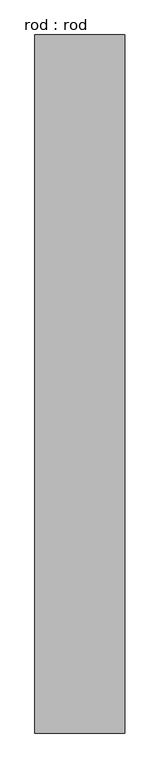
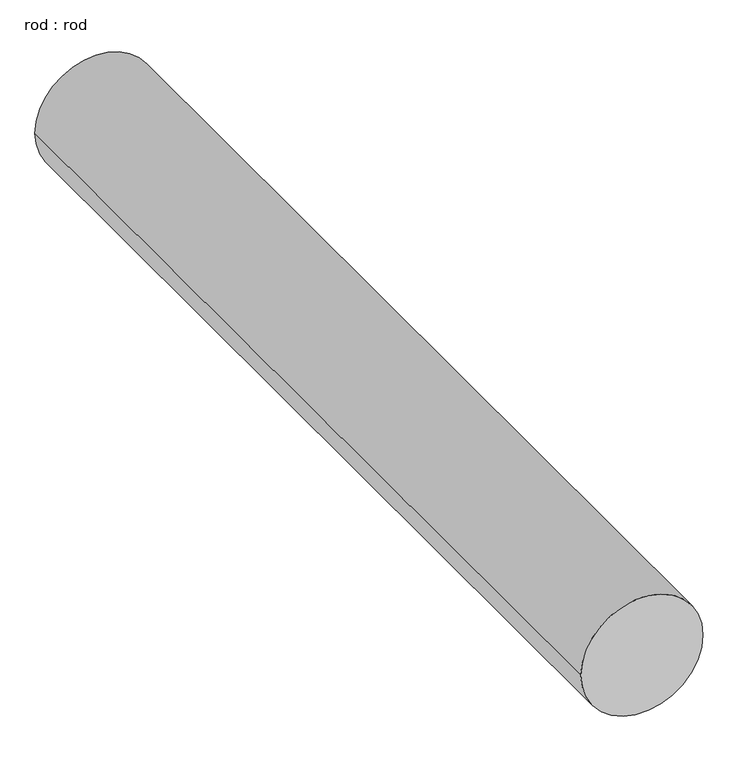
"""IFC4 building model written with IfcOpenShell, lengths in millimetres: proxy geometry, rod : rod."""

from ifc_helpers import new_model, si_unit, point, frame, frame_2d, origin, place, context, project, spatial, circle_curve, trimmed, segment, composite_curve, outline, extrude, source, transform, mapped, element, save


def rod_rod_de65b9e6(model_context):
    return source(origin(), model_context, "Body", "SweptSolid", [
        extrude(outline(composite_curve([segment(trimmed(circle_curve(frame_2d((0.0108462, 0.0)), 200.0), [point((0.0108462, 200.0))], [point((0.0108462, -200.0))], False, "CARTESIAN"), True, "CONTINUOUS"), segment(trimmed(circle_curve(frame_2d((0.0108462, 0.0)), 200.0), [point((0.0108462, -200.0))], [point((0.0108462, 200.0))], False, "CARTESIAN"), True, "CONTINUOUS")], self_intersect=False)), frame((0.0, 2542.7286153, 0.0), z_axis=(0.0, 1.0, 0.0), x_axis=(0.0, 0.0, 1.0)), (0.0, 0.0, 1.0), 3100.0),
    ])


if __name__ == "__main__":
    model = new_model("IFC4")
    model_context = context("Model", 3, world=origin())
    ifc_project = project(units=[si_unit("LENGTHUNIT", "METRE", prefix="MILLI")], contexts=[model_context])
    site = spatial("IfcSite", under=ifc_project)
    building = spatial("IfcBuilding", under=site)
    placement = place(None, origin())
    rod_rod_shape = rod_rod_de65b9e6(model_context)
    element("IfcBuildingElementProxy", 1, Name="rod : rod", ObjectType="rod : rod", at=placement, inside=building, context=model_context, shape_type="MappedRepresentation", body=[
        mapped(rod_rod_shape, transform((0.0, 0.0, 0.0), x_axis=(1.0, 0.0, 0.0), y_axis=(0.0, 1.0, 0.0), z_axis=(0.0, 0.0, 1.0))),
    ])
    save(model, "model.ifc")

# Revit data of these elements
# Type "rod : rod"
#   Default Elevation = 0
